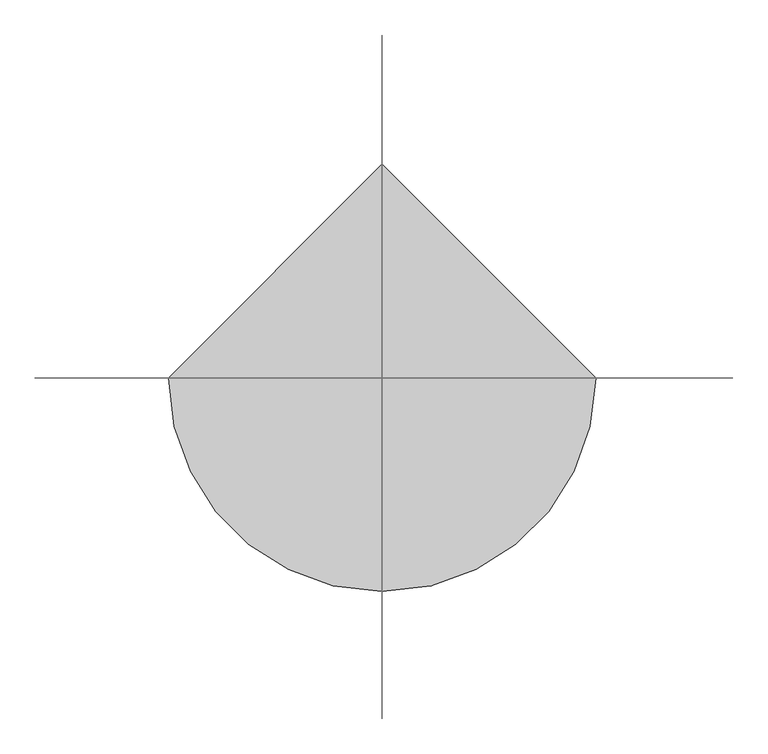
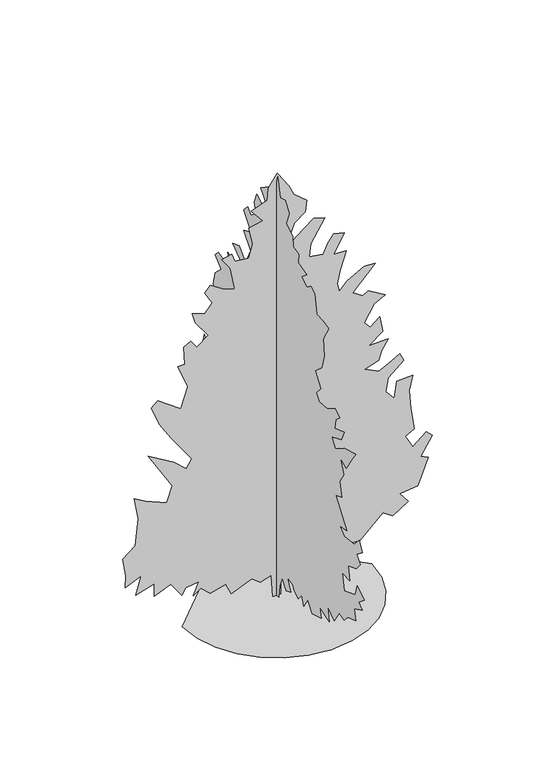
"""IFC4 building model written with IfcOpenShell, lengths in millimetres: proxy geometry, holly miniature 26078 : holly miniature 26078."""

from ifc_helpers import new_model, si_unit, origin, place, context, project, spatial, triangles, source, transform, mapped, element, save


def entourage_9c913b6c(model_context):
    return source(origin(), model_context, "Body", "Tessellation", [
        triangles([(6e-07, 14.2176358, 1.67e-05), (3.9e-06, 26.9638997, 91.3171369), (5.3e-06, 55.4926929, 95.2500727), (6.3e-06, 99.9429821, 60.3250469), (1.03e-05, 160.2677792, 104.7750818), (1.07e-05, 192.0178034, 69.850056), (1.31e-05, 220.9545183, 106.6026137), (1.54e-05, 277.7441478, 101.6000848), (1.65e-05, 277.7441478, 136.525106), (2.16e-05, 376.1666831, 161.9251272), (3.77e-05, 611.119384, 349.2502665), (4.08e-05, 623.8168648, 431.8003512), (3.82e-05, 538.0918284, 476.2503633), (3.59e-05, 468.2417679, 501.6504118), (4.11e-05, 522.21678, 596.9004845), (4.62e-05, 588.8918527, 666.7505087), (4.6e-05, 534.9168042, 739.7755571), (4.75e-05, 515.8668042, 819.150654), (4.39e-05, 468.2417679, 771.5255814), (4.05e-05, 395.2166831, 765.1756056), (4.39e-05, 433.3167194, 822.3256783), (4.03e-05, 338.0691902, 844.5507025), (4.63e-05, 385.6916831, 974.7257509), (5.23e-05, 452.3667558, 1076.325872), (5.33e-05, 436.4917437, 1133.475872), (5.27e-05, 395.2166831, 1174.7509689), (5.57e-05, 436.4917437, 1212.8509689), (5.55e-05, 417.4442508, 1235.0759205), (5.08e-05, 328.5416468, 1212.8509689), (5.36e-05, 347.5916468, 1276.3510174), (4.79e-05, 255.5191236, 1222.3759689), (4.96e-05, 249.1678579, 1289.0509689), (5.38e-05, 312.6666347, 1336.6761143), (5.23e-05, 268.2165862, 1352.5510174), (4.99e-05, 236.4678337, 1320.8010658), (4.67e-05, 188.8427974, 1282.7010658), (4.91e-05, 204.7178095, 1339.8510658), (4.95e-05, 185.6677913, 1381.1261627), (5.34e-05, 233.2928277, 1441.4511143), (5.18e-05, 182.4928034, 1463.6762112), (5.6e-05, 233.2928277, 1530.3512112), (5.58e-05, 207.8928155, 1558.9262112), (5.41e-05, 185.6677913, 1536.7012596), (5.33e-05, 147.5677641, 1568.4512112), (5.5e-05, 160.2677792, 1606.5513565), (5.56e-05, 141.217761, 1654.1763565), (5.22e-05, 87.2427217, 1619.2513081), (5.18e-05, 65.017702, 1641.4762596), (5.57e-05, 112.6427429, 1698.626405), (5.41e-05, 49.1426899, 1743.0764534), (5.31e-05, 7.8675799, 1768.4763565), (5.39e-05, -8.0073817, 1819.2764534), (5.08e-05, -22.8780526, 1737.2217236), (4.95e-05, -58.8071436, 1749.4263565), (4.7e-05, -87.3824206, 1708.151405), (4.62e-05, -68.3324025, 1654.1763565), (4.34e-05, -112.7824418, 1625.6013565), (4.19e-05, -115.9574388, 1581.1513081), (3.99e-05, -157.2324812, 1574.8012596), (3.9e-05, -150.8824691, 1533.5261627), (3.58e-05, -211.2075115, 1517.6512596), (3.65e-05, -176.2824994, 1489.0762596), (3.42e-05, -211.2075115, 1463.6762112), (3.36e-05, -239.7825478, 1485.9011627), (3.18e-05, -271.5338438, 1473.2012112), (2.87e-05, -284.2338498, 1390.6511627), (2.66e-05, -331.8588861, 1390.6511627), (2.46e-05, -369.9589225, 1381.1261627), (2.43e-05, -331.8588861, 1314.4510174), (2.19e-05, -338.2088983, 1241.4259689), (2.09e-05, -319.1588619, 1181.1009447), (2.17e-05, -274.7088316, 1139.8259205), (1.84e-05, -312.8088861, 1085.850872), (1.87e-05, -281.0588438, 1047.750872), (1.69e-05, -303.283868, 1022.3508236), (1.46e-05, -357.6551313, 1025.5435793), (1.31e-05, -414.4089346, 1060.4508236), (1.11e-05, -446.1589588, 1041.4008236), (1.15e-05, -420.7589467, 1016.0008478), (1.07e-05, -411.2314033, 974.7257509), (8.3e-06, -477.9090194, 996.9507751), (7.9e-06, -458.858983, 952.5007267), (1.01e-05, -389.0089225, 923.9257267), (7.9e-06, -415.6357856, 888.360601), (6.2e-06, -481.0840073, 930.2757751), (3.3e-06, -560.4590678, 952.5007267), (3.4e-06, -531.8840315, 911.2257025), (3.3e-06, -493.7840315, 850.9006783), (5.8e-06, -449.333983, 869.9506783), (2.9e-06, -477.0326921, 812.787961), (2.9e-06, -446.1564517, 765.1756056), (4e-07, -462.0340073, 704.8505814), (1.7e-06, -420.7589467, 688.9755329), (-4.9e-06, -496.9564759, 581.0254724), (-2.9e-06, -446.1564517, 571.5004724), (-5.1e-06, -477.9090194, 546.1004239), (-8.1e-06, -550.9340678, 555.6254602), (-8.5e-06, -585.8590799, 593.7254602), (-1.07e-05, -608.0841042, 552.450436), (-9.8e-06, -566.8090799, 520.7004118), (-1.18e-05, -592.209092, 492.1254118), (-1.16e-05, -563.6340557, 457.2003633), (-9.7e-06, -506.4840194, 434.9753391), (-1.19e-05, -519.1840436, 377.8253028), (-9.5e-06, -465.8973252, 379.8446199), (-1.22e-05, -481.0814638, 311.1502665), (-1.48e-05, -557.2840799, 339.7252665), (-1.39e-05, -569.9840678, 387.3503028), (-1.72e-05, -620.7841284, 355.6002786), (-1.64e-05, -582.684092, 323.8502543), (-1.81e-05, -608.0841042, 304.8002543), (-1.64e-05, -550.9340678, 276.225218), (-1.82e-05, -560.4590678, 228.6001817), (-1.63e-05, -503.306488, 209.5501635), (-1.6e-05, -477.9090194, 180.9751453), (-1.41e-05, -442.9839709, 190.5001453), (-1.42e-05, -408.0564154, 136.525106), (-1.11e-05, -360.4339225, 168.2751393), (-1.34e-05, -373.1313669, 111.1250848), (-9.7e-06, -306.458874, 133.350109), (-1.14e-05, -315.9813306, 92.0750757), (-9.1e-06, -252.4825539, 73.0250575), (-6.5e-06, -220.7325296, 114.3000908), (-6.5e-06, -192.1575115, 69.850056), (-4.7e-06, -176.2824994, 107.9500878), (-4.5e-06, -150.8824691, 76.2000636), (-2.8e-06, -125.4824479, 95.2500727), (-1.6e-06, -112.7824418, 114.3000908), (4e-07, -74.68241, 123.8250999), (-2.3e-06, -100.0824267, 73.0250575), (-1.3e-06, -68.3324025, 60.3250469), (1.2e-06, -39.7573798, 98.4250787), (7e-07, -20.0124481, 53.1848487), (-6e-07, -14.3573869, 1.58e-05), (-16.1742762, 3.5e-06, 1.68e-05), (-22.5242565, -5e-07, 95.2500727), (-66.9742641, 1.5e-06, 79.3750606), (-101.8992944, 1.2e-06, 107.9500878), (-187.6243579, 5.4e-06, 73.0250575), (-209.8493822, 3.9e-06, 120.6500939), (-273.3499393, 6.5e-06, 104.7750818), (-311.4499575, 6.1e-06, 139.700112), (-343.1999817, 8e-06, 117.4750969), (-320.9749938, 4.9e-06, 171.4501453), (-372.9815214, 6.8e-06, 163.8728099), (-390.825018, 8.6e-06, 136.525106), (-435.2750665, 7.1e-06, 200.0251635), (-501.9501391, 1.71e-05, 171.4501453), (-501.9501391, 7.9e-06, 225.4251756), (-578.1501755, 1.8e-05, 203.2001696), (-555.9251513, 7.1e-06, 279.4002241), (-622.6002239, 1.72e-05, 250.8252059), (-619.4251997, 1.48e-05, 301.6252483), (-632.1252239, 5e-06, 377.8253028), (-581.3251997, 1.6e-06, 419.100327), (-568.6251755, -3.7e-06, 530.2254118), (-584.5001876, -7.4e-06, 622.3005329), (-540.0501391, -7.6e-06, 596.9004845), (-451.1500786, -8.5e-06, 558.8004481), (-428.9250544, -1.9e-05, 625.4754845), (-492.4251028, -2.17e-05, 730.2505571), (-527.3501513, -2.33e-05, 787.4006298), (-422.5750422, -2.35e-05, 723.9005814), (-371.775018, -2.31e-05, 679.4505329), (-349.5499938, -2.53e-05, 714.3755814), (-432.1000786, -2.81e-05, 831.8506783), (-482.9001028, -3.01e-05, 911.2257025), (-514.650127, -3.27e-05, 990.6007994), (-489.2501149, -3.46e-05, 1016.0008478), (-394.0000422, -3.43e-05, 946.1507509), (-365.4250059, -4.58e-05, 1031.8758236), (-406.7000301, -4.91e-05, 1133.475872), (-378.1250301, -5e-05, 1133.475872), (-381.300018, -5.33e-05, 1209.6759447), (-352.725018, -5.49e-05, 1225.5509205), (-327.3249696, -5.41e-05, 1190.6259447), (-280.5940284, -5.71e-05, 1227.0368763), (-333.6749817, -5.87e-05, 1298.5759689), (-346.3750059, -6.03e-05, 1343.0260174), (-295.5749635, -6.1e-05, 1323.9760174), (-263.8249393, -6.36e-05, 1362.0760174), (-295.1355281, -7.18e-05, 1414.3061142), (-273.2864439, -7.37e-05, 1441.3724854), (-216.1993761, -7.37e-05, 1403.3511143), (-171.7493458, -7.44e-05, 1390.6511627), (-190.799364, -7.81e-05, 1485.9011627), (-225.7243943, -7.92e-05, 1533.5261627), (-183.7899808, -8.09e-05, 1543.2950432), (-171.7493458, -7.97e-05, 1508.1262596), (-114.5993004, -8.11e-05, 1501.7762112), (-98.7242883, -8.41e-05, 1558.9262112), (-114.5993004, -8.69e-05, 1631.9512596), (-57.4492595, -9.6e-05, 1644.6513565), (-105.0743004, -9.72e-05, 1701.8013565), (-38.3992414, -0.0001003, 1727.201405), (-35.2242399, -0.0001026, 1778.0013565), (2.8758411, -0.0001061, 1828.8014534), (48.9753037, -0.0001044, 1760.0893684), (69.5505876, -0.0001029, 1714.5013081), (123.5258904, -0.0001026, 1670.051405), (117.1758782, -0.0001002, 1622.4262596), (71.0844965, -9.73e-05, 1587.6612305), (28.2758109, -8.41e-05, 1473.2012112), (79.075851, -9.48e-05, 1527.1762596), (152.1009085, -9.94e-05, 1581.1513081), (196.5509388, -0.0001002, 1568.4512112), (139.4009025, -9.44e-05, 1476.3761627), (133.0508904, -8.5e-05, 1422.4011143), (190.2009449, -9.3e-05, 1412.8761143), (209.250963, -9.55e-05, 1454.1512112), (234.6509751, -9.76e-05, 1485.9011627), (275.9255088, -9.84e-05, 1476.3761627), (234.6509751, -9.37e-05, 1397.0010658), (285.4505088, -9.5e-05, 1393.8261143), (260.0504967, -8.42e-05, 1320.8010658), (247.3509812, -8.13e-05, 1263.6510658), (256.8754907, -8e-05, 1228.7260174), (288.6255149, -8.25e-05, 1263.6510658), (358.4755754, -9.31e-05, 1301.7510658), (402.9255876, -9.43e-05, 1298.5759689), (310.8505391, -8.05e-05, 1203.3259689), (352.1255633, -8.04e-05, 1174.7509689), (374.3505876, -8.18e-05, 1190.6259447), (445.2877547, -8.2e-05, 1148.1927063), (399.7505997, -7.96e-05, 1123.950872), (358.4755754, -7.53e-05, 1057.275872), (383.8755876, -7.48e-05, 1028.7007994), (421.9756239, -7.74e-05, 1060.4508236), (434.6756118, -7.48e-05, 993.7758236), (377.5255754, -7.11e-05, 949.3257751), (456.900636, -7.36e-05, 952.5007267), (431.5006239, -7.1e-05, 911.2257025), (418.8005997, -6.89e-05, 873.1257025), (361.6505633, -6.64e-05, 854.0757025), (418.8005997, -6.68e-05, 825.5006298), (457.6550231, -6.87e-05, 843.1206299), (504.5256723, -7.13e-05, 869.9506783), (520.4006845, -7.04e-05, 838.200654), (456.900636, -6.61e-05, 784.2256056), (447.375636, -6.32e-05, 727.0756056), (482.3006481, -6.24e-05, 685.8005814), (491.8256845, -6.58e-05, 755.6506056), (558.5007208, -6.8e-05, 758.8256298), (542.6257087, -6.48e-05, 698.5005329), (548.9757208, -6.14e-05, 619.1255087), (564.8507329, -5.08e-05, 523.875436), (526.7506966, -4.89e-05, 504.8253997), (558.5007208, -4.72e-05, 447.6753633), (612.4757692, -5.1e-05, 495.3003997), (637.8758177, -5.06e-05, 469.9003876), (590.250745, -4.59e-05, 396.8753028), (622.0007692, -4.62e-05, 381.0002907), (577.5507571, -4e-05, 273.050212), (504.5256723, -3.74e-05, 263.525212), (539.4507208, -3.65e-05, 219.0751817), (475.9506723, -2.59e-05, 177.8001393), (434.6756118, -2.6e-05, 206.3751575), (339.4255391, -1.91e-05, 117.4750969), (291.8005209, -1.79e-05, 120.6500939), (215.600957, -1.33e-05, 69.850056), (164.8009146, -1.38e-05, 114.3000908), (120.3508843, -4e-06, 76.2000636), (88.6008601, -3.7e-06, 92.0750757), (47.3258268, -4e-07, 44.4500348), (18.7507268, -2.3e-06, 107.9500878), (15.5757242, 2.6e-06, 1.58e-05), (-388.6203197, 1e-06, 2.79e-05), (-378.3460196, -89.0461181, 2.49e-05), (-349.0877037, -170.8207325, 2.16e-05), (-303.1848006, -242.9809173, 1.81e-05), (-242.9809173, -303.1848006, 1.45e-05), (-170.8207325, -349.0877037, 1.1e-05), (-89.0461181, -378.3460196, 7.7e-06), (1.7e-05, -388.6203197, 4.7e-06), (89.0461181, -378.3460196, 2.3e-06), (170.8207325, -349.0877037, 8e-07), (242.9809173, -303.1848006, 0.0), (303.1848006, -242.9809173, 0.0), (349.0877037, -170.8207325, 8e-07), (378.3460196, -89.0461181, 2.3e-06), (388.6203197, 3.91e-05, 4.7e-06), (-5.1e-05, 388.6203197, 2.79e-05)], [[51, 52, 53], [85, 86, 87], [29, 30, 31], [80, 81, 82], [80, 82, 83], [60, 61, 62], [123, 124, 125], [32, 33, 34], [32, 34, 35], [17, 18, 19], [118, 119, 120], [110, 111, 112], [93, 94, 95], [20, 21, 22], [97, 98, 99], [97, 99, 100], [108, 109, 110], [107, 108, 110], [32, 35, 36], [67, 68, 69], [103, 104, 105], [38, 39, 40], [77, 78, 79], [76, 77, 79], [85, 87, 88], [85, 88, 89], [84, 85, 89], [45, 46, 47], [5, 6, 7], [44, 45, 47], [7, 8, 9], [48, 49, 50], [129, 130, 131], [129, 131, 132], [76, 79, 80], [41, 42, 43], [40, 41, 43], [107, 110, 112], [106, 107, 112], [116, 117, 118], [31, 32, 36], [58, 59, 60], [66, 67, 69], [125, 126, 127], [26, 27, 28], [26, 28, 29], [120, 121, 122], [120, 122, 123], [133, 134, 1], [133, 1, 2], [132, 133, 2], [91, 92, 93], [112, 113, 114], [106, 112, 114], [100, 101, 102], [15, 16, 17], [50, 51, 53], [48, 50, 53], [72, 73, 74], [3, 4, 5], [53, 54, 55], [53, 55, 56], [48, 53, 56], [96, 97, 100], [96, 100, 102], [96, 102, 103], [11, 12, 13], [10, 11, 13], [10, 13, 14], [125, 127, 128], [76, 80, 83], [75, 76, 83], [15, 17, 19], [15, 19, 20], [14, 15, 20], [114, 115, 116], [106, 114, 116], [9, 10, 14], [63, 64, 65], [63, 65, 66], [89, 90, 91], [84, 89, 91], [106, 116, 118], [56, 57, 58], [48, 56, 58], [47, 48, 58], [40, 43, 44], [105, 106, 118], [96, 103, 105], [95, 96, 105], [44, 47, 58], [40, 44, 58], [40, 58, 60], [38, 40, 60], [38, 60, 62], [38, 62, 63], [38, 63, 66], [37, 38, 66], [36, 37, 66], [36, 66, 69], [36, 69, 70], [36, 70, 71], [36, 71, 72], [36, 72, 74], [31, 36, 74], [23, 24, 25], [23, 25, 26], [23, 26, 29], [23, 29, 31], [23, 31, 74], [22, 23, 74], [22, 74, 75], [22, 75, 83], [22, 83, 84], [22, 84, 91], [22, 91, 93], [22, 93, 95], [20, 22, 95], [14, 20, 95], [9, 14, 95], [7, 9, 95], [5, 7, 95], [3, 5, 95], [2, 3, 95], [132, 2, 95], [129, 132, 95], [129, 95, 105], [129, 105, 118], [128, 129, 118], [125, 128, 118], [123, 125, 118], [120, 123, 118], [161, 162, 163], [142, 143, 144], [219, 220, 221], [218, 219, 221], [156, 157, 158], [178, 179, 180], [160, 161, 163], [160, 163, 164], [230, 231, 232], [149, 150, 151], [223, 224, 225], [227, 228, 229], [217, 218, 221], [151, 152, 153], [263, 264, 265], [147, 148, 149], [186, 187, 188], [186, 188, 189], [171, 172, 173], [145, 146, 147], [196, 197, 198], [193, 194, 195], [227, 229, 230], [242, 243, 244], [241, 242, 244], [205, 206, 207], [204, 205, 207], [213, 214, 215], [222, 223, 225], [211, 212, 213], [210, 211, 213], [209, 210, 213], [195, 196, 198], [241, 244, 245], [254, 255, 256], [254, 256, 257], [236, 237, 238], [236, 238, 239], [235, 236, 239], [177, 178, 180], [156, 158, 159], [191, 192, 193], [265, 266, 135], [265, 135, 136], [138, 139, 140], [203, 204, 207], [203, 207, 208], [248, 249, 250], [248, 250, 251], [195, 198, 199], [251, 252, 253], [182, 183, 184], [181, 182, 184], [193, 195, 199], [174, 175, 176], [173, 174, 176], [168, 169, 170], [167, 168, 170], [166, 167, 170], [251, 253, 254], [222, 225, 226], [259, 260, 261], [230, 232, 233], [230, 233, 234], [245, 246, 247], [155, 156, 159], [193, 199, 200], [193, 200, 201], [193, 201, 202], [191, 193, 202], [191, 202, 203], [190, 191, 203], [261, 262, 263], [248, 251, 254], [151, 153, 154], [151, 154, 155], [136, 137, 138], [181, 184, 185], [140, 141, 142], [140, 142, 144], [241, 245, 247], [186, 189, 190], [185, 186, 190], [185, 190, 203], [165, 166, 170], [151, 155, 159], [149, 151, 159], [147, 149, 159], [145, 147, 159], [144, 145, 159], [221, 222, 226], [235, 239, 240], [209, 213, 215], [209, 215, 216], [208, 209, 216], [171, 173, 176], [177, 180, 181], [177, 181, 185], [185, 203, 208], [185, 208, 216], [177, 185, 216], [177, 216, 217], [234, 235, 240], [140, 144, 159], [138, 140, 159], [138, 159, 160], [138, 160, 164], [138, 164, 165], [136, 138, 165], [265, 136, 165], [257, 258, 259], [217, 221, 226], [177, 217, 226], [176, 177, 226], [171, 176, 226], [170, 171, 226], [165, 170, 226], [265, 165, 226], [265, 226, 227], [265, 227, 230], [265, 230, 234], [265, 234, 240], [263, 265, 240], [261, 263, 240], [259, 261, 240], [257, 259, 240], [257, 240, 241], [257, 241, 247], [254, 257, 247], [248, 254, 247], [281, 282, 267], [280, 281, 267], [280, 267, 268], [279, 280, 268], [279, 268, 269], [279, 269, 270], [278, 279, 270], [277, 278, 270], [277, 270, 271], [277, 271, 272], [277, 272, 273], [277, 273, 274], [277, 274, 275], [277, 275, 276]], closed=False),
    ])


if __name__ == "__main__":
    model = new_model("IFC4")
    model_context = context("Model", 3, world=origin())
    ifc_project = project(units=[si_unit("LENGTHUNIT", "METRE", prefix="MILLI")], contexts=[model_context])
    site = spatial("IfcSite", under=ifc_project)
    building = spatial("IfcBuilding", under=site)
    placement = place(None, origin())
    entourage_shape = entourage_9c913b6c(model_context)
    element("IfcBuildingElementProxy", 1, Name="holly miniature 26078 : holly miniature 26078", ObjectType="holly miniature 26078 : holly miniature 26078", at=placement, inside=building, context=model_context, shape_type="MappedRepresentation", body=[
        mapped(entourage_shape, transform((0.0, 0.0, 0.0), x_axis=(1.0, 0.0, 0.0), y_axis=(0.0, 1.0, 0.0), z_axis=(0.0, 0.0, 1.0))),
    ])
    save(model, "model.ifc")

# Revit data of these elements
# Type "holly miniature 26078 : holly miniature 26078"
#   built-in parameter 1005195 = "RPC-16-FXGU-6LXX-PKLL-J000-ST1L-LVER-AU"
#   Height = 0
